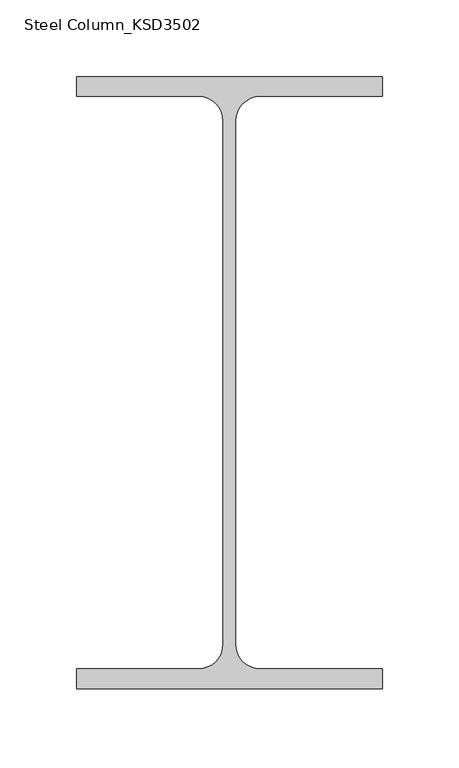
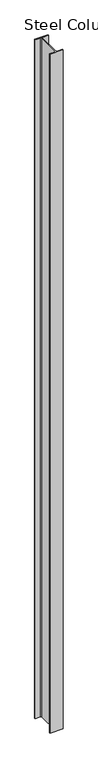
"""IFC4 building model written with IfcOpenShell, lengths in millimetres: column geometry, Steel Column_KSD3502 : H_SC_ASC_H-400×200x8x13."""

from ifc_helpers import new_model, si_unit, point, frame, frame_2d, origin, place, context, project, spatial, polyline, circle_curve, trimmed, segment, composite_curve, outline, extrude, source, transform, mapped, element, save


def steel_column_ksd3502_8add4d16(model_context):
    return source(origin(), model_context, "Body", "SweptSolid", [
        extrude(outline(composite_curve([segment(polyline([(100.0, 200.0), (100.0, 187.0), (20.0, 187.0)]), True, "CONTINUOUS"), segment(trimmed(circle_curve(frame_2d((20.0, 171.0)), 16.0), [point((20.0, 187.0))], [point((4.0, 171.0))], True, "CARTESIAN"), True, "CONTINUOUS"), segment(polyline([(4.0, 171.0), (4.0, -171.0)]), True, "CONTINUOUS"), segment(trimmed(circle_curve(frame_2d((20.0, -171.0)), 16.0), [point((4.0, -171.0))], [point((20.0, -187.0))], True, "CARTESIAN"), True, "CONTINUOUS"), segment(polyline([(20.0, -187.0), (100.0, -187.0), (100.0, -200.0), (-100.0, -200.0), (-100.0, -187.0), (-20.0, -187.0)]), True, "CONTINUOUS"), segment(trimmed(circle_curve(frame_2d((-20.0, -171.0)), 16.0), [point((-20.0, -187.0))], [point((-4.0, -171.0))], True, "CARTESIAN"), True, "CONTINUOUS"), segment(polyline([(-4.0, -171.0), (-4.0, 171.0)]), True, "CONTINUOUS"), segment(trimmed(circle_curve(frame_2d((-20.0, 171.0)), 16.0), [point((-4.0, 171.0))], [point((-20.0, 187.0))], True, "CARTESIAN"), True, "CONTINUOUS"), segment(polyline([(-20.0, 187.0), (-100.0, 187.0), (-100.0, 200.0), (100.0, 200.0)]), True, "CONTINUOUS")], self_intersect=False)), frame((0.0, 0.0, 7249.9720055), z_axis=(0.0, 0.0, 1.0), x_axis=(1.0, 0.0, 0.0)), (0.0, 0.0, 1.0), 10950.0),
    ])


if __name__ == "__main__":
    model = new_model("IFC4")
    model_context = context("Model", 3, world=origin())
    ifc_project = project(units=[si_unit("LENGTHUNIT", "METRE", prefix="MILLI")], contexts=[model_context])
    site = spatial("IfcSite", under=ifc_project)
    building = spatial("IfcBuilding", under=site)
    placement = place(None, origin())
    steel_column_ksd3502_shape = steel_column_ksd3502_8add4d16(model_context)
    element("IfcColumn", 1, ObjectType="Steel Column_KSD3502 : H_SC_ASC_H-400×200x8x13", at=placement, inside=building, context=model_context, shape_type="MappedRepresentation", body=[
        mapped(steel_column_ksd3502_shape, transform((0.0, 0.0, 0.0), x_axis=(1.0, 0.0, 0.0), y_axis=(0.0, 1.0, 0.0), z_axis=(0.0, 0.0, 1.0))),
    ])
    save(model, "model.ifc")

# Revit data of these elements
# Type "Steel Column_KSD3502 : H_SC_ASC_H-400×200x8x13"
#   Width = 20.0 cm
#   Web Thickness = 0.8 cm
#   Web Fillet = 1.6 cm
#   Warping Constant = 648999.0 cm⁶
#   Torsional Moment of Inertia = 35.8981 cm⁴
#   Section Area = 84.12 cm²
#   Plastic Modulus weak axis = 268.0 cm³
#   Plastic Modulus strong axis = 1330.0 cm³
#   Perimeter = 1.27 m²/m
#   Nominal Weight = 66.00 kgf/m
#   Moment of Inertia weak axis = 1740.00 cm⁴
#   Moment of Inertia strong axis = 23700.00 cm⁴
#   Height = 40.0 cm
#   Flange Thickness = 1.3 cm
#   Elastic Modulus weak axis = 174.0 cm³
#   Elastic Modulus strong axis = 1190.0 cm³
#   Centroid Vertical = 20.0 cm
#   Centroid Horizontal = 10.0 cm
#   Bolt Spacing = 13.97 cm
#   Structural Material [instance default] = Steel, 45-345
#   Section Name Key = ""
#   Assembly Code = ""
# Element 1 (IfcColumn, "Steel Column_KSD3502 : H_SC_ASC_H-400×200x8x13")
#   Structural Material = none
# Materials
#   "Steel, 45-345": class "Metal", colour RGB 189 187 185, transparency 0, Description = "Steel 345 MPa", Cost = 0
